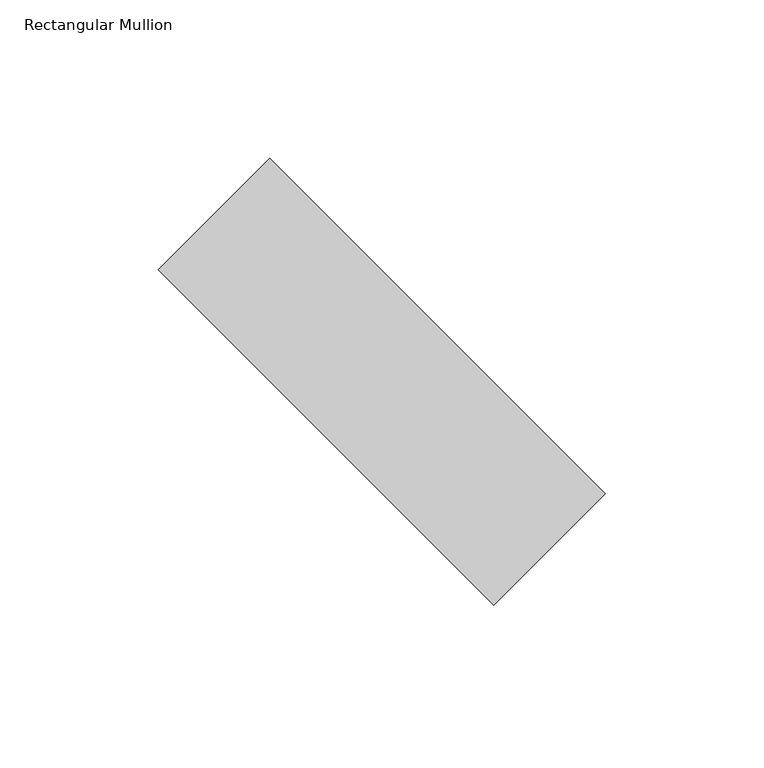
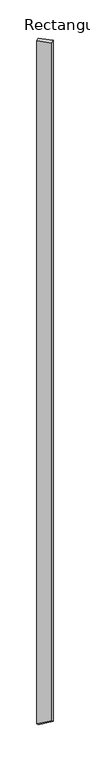
"""IFC4 building model written with IfcOpenShell, lengths in millimetres: member geometry, Rectangular Mullion : tilted mullions."""

from ifc_helpers import new_model, si_unit, origin, place, context, project, spatial, faceted_brep, source, transform, mapped, element, save


def rectangular_mullion_aeb8e4f0(model_context):
    return source(origin(), model_context, "Body", "Brep", [
        faceted_brep([(-35.3553391, 70.7106781, 0.0), (-70.7106781, 35.3553391, 0.0), (35.3553391, -70.7106781, 0.0), (70.7106781, -35.3553391, 0.0), (-35.3553391, 70.7106781, -8054.7810851), (-70.7106781, 35.3553391, -8009.722691), (35.3553391, -70.7106781, -7944.7021553), (70.7106781, -35.3553391, -7989.7605495)], [[[0, 1, 2, 3]], [[1, 0, 4, 5]], [[2, 1, 5, 6]], [[3, 2, 6, 7]], [[0, 3, 7, 4]], [[4, 7, 6, 5]]]),
    ])


if __name__ == "__main__":
    model = new_model("IFC4")
    model_context = context("Model", 3, world=origin())
    ifc_project = project(units=[si_unit("LENGTHUNIT", "METRE", prefix="MILLI")], contexts=[model_context])
    site = spatial("IfcSite", under=ifc_project)
    building = spatial("IfcBuilding", under=site)
    placement = place(None, origin())
    rectangular_mullion_shape = rectangular_mullion_aeb8e4f0(model_context)
    element("IfcMember", 1, ObjectType="Rectangular Mullion : tilted mullions", at=placement, inside=building, context=model_context, shape_type="MappedRepresentation", body=[
        mapped(rectangular_mullion_shape, transform((0.0, 0.0, 0.0), x_axis=(1.0, 0.0, 0.0), y_axis=(0.0, 1.0, 0.0), z_axis=(0.0, 0.0, 1.0))),
    ])
    save(model, "model.ifc")

# Revit data of these elements
# Type "Rectangular Mullion : tilted mullions"
#   built-in parameter 1007304 = 0.492126 (stored number, unit not read)
#   built-in parameter 1007301 = 0.082021 (stored number, unit not read)
#   built-in parameter 1007300 = 0.082021 (stored number, unit not read)
# Element 1 (IfcMember, "Rectangular Mullion : tilted mullions")
#   Materials on its faces: "Aluminum"
# Materials
#   "Aluminum": class "Metal", colour RGB 244 244 244, transparency 0, Description = "Aluminum 6061", Cost = 0
